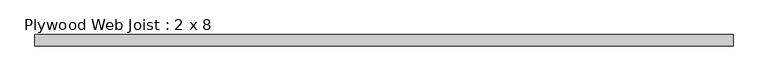
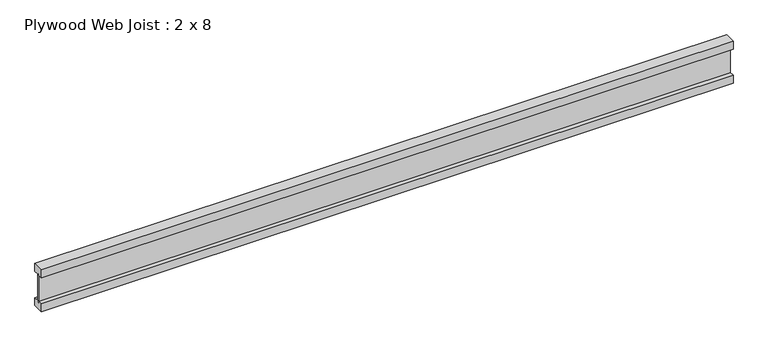
"""IFC4 building model written with IfcOpenShell, lengths in millimetres: beam geometry, Plywood Web Joist : 2 x 8."""

from ifc_helpers import new_model, si_unit, frame, origin, place, context, project, spatial, polyline, outline, extrude, source, transform, mapped, element, save


def plywood_web_joist_2_x_8_5f52603e(model_context):
    return source(origin(), model_context, "Body", "SweptSolid", [
        extrude(outline(polyline([(-25.4, 101.6), (25.4, 101.6), (25.4, 63.5), (4.7625, 63.5), (4.7625, 69.85), (-4.7625, 69.85), (-4.7625, 63.5), (-25.4, 63.5), (-25.4, 101.6)])), frame((-1584.325, 0.0, 0.0), z_axis=(1.0, 0.0, 0.0), x_axis=(0.0, 1.0, 0.0)), (0.0, 0.0, 1.0), 3168.65),
        extrude(outline(polyline([(25.4, -63.5), (25.4, -101.6), (-25.4, -101.6), (-25.4, -63.5), (-4.7625, -63.5), (-4.7625, -69.1160374), (4.7625, -69.1160374), (4.7625, -63.5), (25.4, -63.5)])), frame((-1584.325, 0.0, 0.0), z_axis=(1.0, 0.0, 0.0), x_axis=(0.0, 1.0, 0.0)), (0.0, 0.0, 1.0), 3168.65),
        extrude(outline(polyline([(1584.325, 4.7625), (1584.325, -4.7625), (-1584.325, -4.7625), (-1584.325, 4.7625), (1584.325, 4.7625)])), frame((0.0, 0.0, -69.1160374), z_axis=(0.0, 0.0, 1.0), x_axis=(1.0, 0.0, 0.0)), (0.0, 0.0, 1.0), 138.9660374),
    ])


if __name__ == "__main__":
    model = new_model("IFC4")
    model_context = context("Model", 3, world=origin())
    ifc_project = project(units=[si_unit("LENGTHUNIT", "METRE", prefix="MILLI")], contexts=[model_context])
    site = spatial("IfcSite", under=ifc_project)
    building = spatial("IfcBuilding", under=site)
    placement = place(None, origin())
    plywood_web_joist_2_x_8_shape = plywood_web_joist_2_x_8_5f52603e(model_context)
    element("IfcBeam", 1, ObjectType="Plywood Web Joist : 2 x 8", at=placement, inside=building, context=model_context, shape_type="MappedRepresentation", body=[
        mapped(plywood_web_joist_2_x_8_shape, transform((0.0, 0.0, 0.0), x_axis=(1.0, 0.0, 0.0), y_axis=(0.0, 1.0, 0.0), z_axis=(0.0, 0.0, 1.0))),
    ])
    save(model, "model.ifc")

# Revit data of these elements
# Type "Plywood Web Joist : 2 x 8"
#   Assembly Code = "B10"
#   Length [instance default] = 5' - 0"
#   b = 0' - 2"
#   d = 0' - 8"
#   Structural Material [instance default] = Softwood, Lumber
# Element 1 (IfcBeam, "Plywood Web Joist : 2 x 8")
#   Materials on its faces: "Softwood, Lumber"
# Materials
#   "Softwood, Lumber": class "Wood", colour RGB 144 113 62, transparency 0, Description = "Pinus Echinata", Cost = 0
